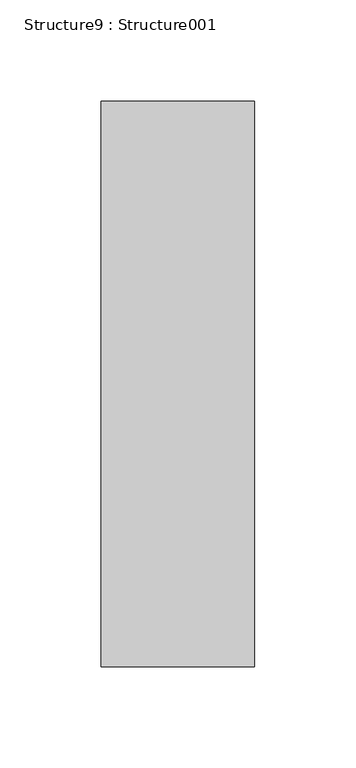
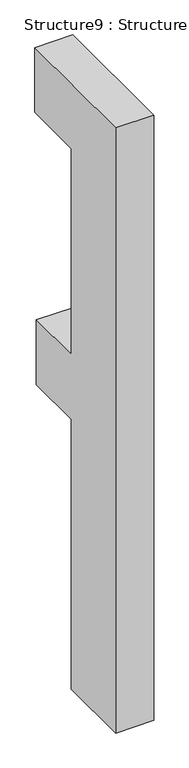
"""IFC4 building model written with IfcOpenShell, lengths in millimetres: proxy geometry, Structure9 : Structure001."""

from ifc_helpers import new_model, si_unit, frame, origin, place, context, project, spatial, polyline, outline, extrude, source, transform, mapped, element, save


def structure9_structure001_6030518d(model_context):
    return source(origin(), model_context, "Body", "SweptSolid", [
        extrude(outline(polyline([(1280.4310236, 0.0), (1280.4310236, -279.8753697), (1143.2462515, -279.8753697), (1143.2462515, -153.6692086), (707.9014148, -153.6692086), (707.9014148, -274.4042785), (570.7022407, -274.4042785), (570.7022407, -153.6692086), (0.0, -153.6692086), (0.0, 0.0), (1280.4310236, 0.0)])), frame((-35624.0862846, 276682.2393327, 4479.6663888), z_axis=(1.0, 0.0, 1.354250045437766e-12), x_axis=(-1.354250045437766e-12, 0.0, 1.0)), (0.0, 0.0, 1.0), 76.2),
    ])


if __name__ == "__main__":
    model = new_model("IFC4")
    model_context = context("Model", 3, world=origin())
    ifc_project = project(units=[si_unit("LENGTHUNIT", "METRE", prefix="MILLI")], contexts=[model_context])
    site = spatial("IfcSite", under=ifc_project)
    building = spatial("IfcBuilding", under=site)
    placement = place(None, origin())
    structure9_structure001_shape = structure9_structure001_6030518d(model_context)
    element("IfcBuildingElementProxy", 1, Name="Structure9 : Structure001", ObjectType="Structure9 : Structure001", at=placement, inside=building, context=model_context, shape_type="MappedRepresentation", body=[
        mapped(structure9_structure001_shape, transform((0.0, 0.0, 0.0), x_axis=(1.0, 0.0, 0.0), y_axis=(0.0, 1.0, 0.0), z_axis=(0.0, 0.0, 1.0))),
    ])
    save(model, "model.ifc")

# Revit data of these elements
# Type "Structure9 : Structure001"
#   NameOverride = "Structure001"
# Element 1 (IfcBuildingElementProxy, "Structure9 : Structure001")
#   Materials on its faces: "BRUSHED ALUMINUM LETTERING"
# Materials
#   "BRUSHED ALUMINUM LETTERING": class "Unassigned", colour RGB 169 181 186, transparency 0, Cost = 0
